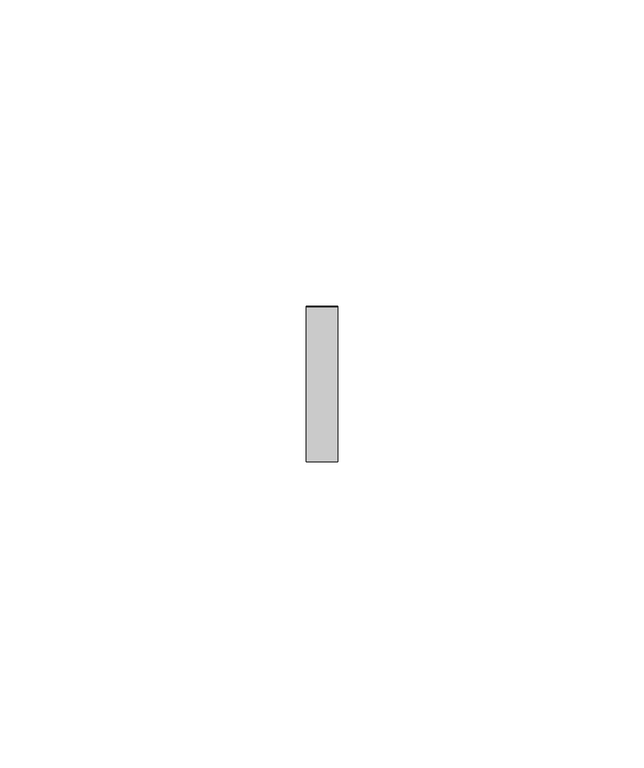
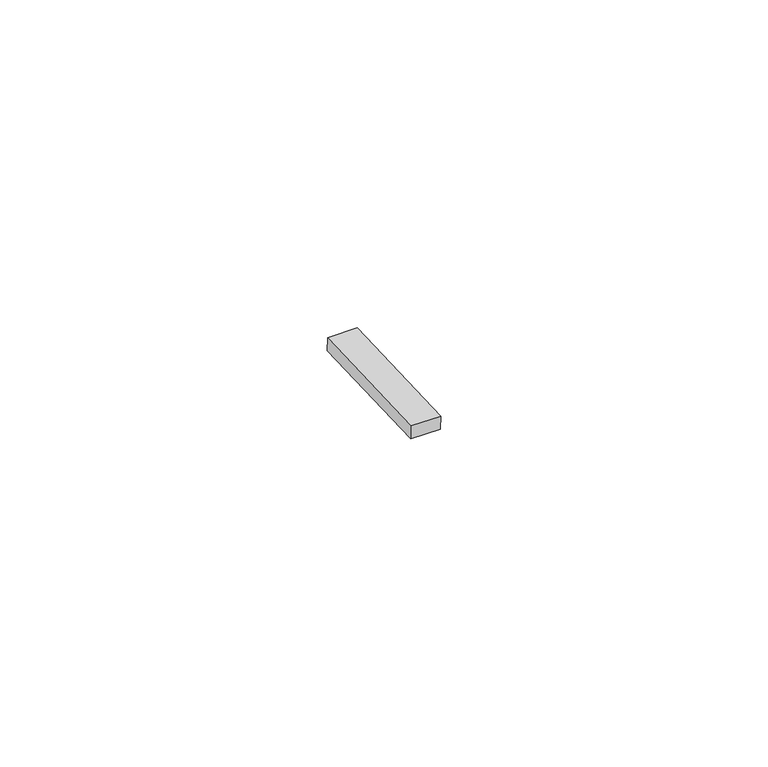
"""IFC4 building model written with IfcOpenShell, lengths in millimetres: proxy geometry, Inner panel:Inner panel:1:Inner panel:1 : Inner panel:Inner panel:300324:2:Inner panel:1:Inner panel:1 : Inner panel:Inner panel:300324:2 : Inner panel:Inner panel:1:Inner panel:1 : Inner panel:Inner panel:300324:300043:115 : Inner panel:Inner panel:1:Inner panel:1 : Inner panel:Inner panel:300324:2:Inner panel:1:Inner panel:1 : Inner panel:Inner panel:300324:2 : Inner panel:Inner panel:1:Inner panel:1 : Inner panel:Inner panel:300324:300043:308120."""

from ifc_helpers import new_model, si_unit, frame, origin, place, context, project, spatial, polyline, outline, extrude, source, transform, mapped, element, save


def generic_models_5e887ab9(model_context):
    return source(origin(), model_context, "Body", "SweptSolid", [
        extrude(outline(polyline([(0.0, -25.4), (0.0, 0.0), (5.2138089, 0.0), (5.2138089, -25.4), (0.0, -25.4)])), frame((593936.595117, -576574.3073926, 4050.9976844), z_axis=(0.0, -0.041630544712223896, 0.9991330730923502), x_axis=(-1.0, 0.0, 0.0)), (0.0, 0.0, 1.0), 2.4763745),
    ])


if __name__ == "__main__":
    model = new_model("IFC4")
    model_context = context("Model", 3, world=origin())
    ifc_project = project(units=[si_unit("LENGTHUNIT", "METRE", prefix="MILLI")], contexts=[model_context])
    site = spatial("IfcSite", under=ifc_project)
    building = spatial("IfcBuilding", under=site)
    placement = place(None, origin())
    generic_models_shape = generic_models_5e887ab9(model_context)
    element("IfcBuildingElementProxy", 1, Name="Inner panel:Inner panel:1:Inner panel:1 : Inner panel:Inner panel:300324:2:Inner panel:1:Inner panel:1 : Inner panel:Inner panel:300324:2 : Inner panel:Inner panel:1:Inner panel:1 : Inner panel:Inner panel:300324:300043:115 : Inner panel:Inner panel:1:Inner panel:1 : Inner panel:Inner panel:300324:2:Inner panel:1:Inner panel:1 : Inner panel:Inner panel:300324:2 : Inner panel:Inner panel:1:Inner panel:1 : Inner panel:Inner panel:300324:300043:308120", ObjectType="Inner panel:Inner panel:1:Inner panel:1 : Inner panel:Inner panel:300324:2:Inner panel:1:Inner panel:1 : Inner panel:Inner panel:300324:2 : Inner panel:Inner panel:1:Inner panel:1 : Inner panel:Inner panel:300324:300043:115 : Inner panel:Inner panel:1:Inner panel:1 : Inner panel:Inner panel:300324:2:Inner panel:1:Inner panel:1 : Inner panel:Inner panel:300324:2 : Inner panel:Inner panel:1:Inner panel:1 : Inner panel:Inner panel:300324:300043:308120", at=placement, inside=building, context=model_context, shape_type="MappedRepresentation", body=[
        mapped(generic_models_shape, transform((0.0, 0.0, 0.0), x_axis=(1.0, 0.0, 0.0), y_axis=(0.0, 1.0, 0.0), z_axis=(0.0, 0.0, 1.0))),
    ])
    save(model, "model.ifc")

# Revit data of these elements
# Type "Inner panel:Inner panel:1:Inner panel:1 : Inner panel:Inner panel:300324:2:Inner panel:1:Inner panel:1 : Inner panel:Inner panel:300324:2 : Inner panel:Inner panel:1:Inner panel:1 : Inner panel:Inner panel:300324:300043:115 : Inner panel:Inner panel:1:Inner panel:1 : Inner panel:Inner panel:300324:2:Inner panel:1:Inner panel:1 : Inner panel:Inner panel:300324:2 : Inner panel:Inner panel:1:Inner panel:1 : Inner panel:Inner panel:300324:300043:308120"
#   NameOverride = "Inner panel:Inner panel:1:Inner panel:1 : Inner panel:Inner panel:300324:2:Inner panel:1:Inner panel:1 : Inner panel:Inner panel:300324:2 : Inner panel:Inner panel:1:Inner panel:1 : Inner panel:Inner panel:300324:300043:308120"
#   ObjectTypeOverride = "Inner panel:1:Inner panel:1 : Inner panel:Inner panel:300324:2 : Inner panel:Inner panel:1:Inner panel:1 : Inner panel:Inner panel:300324:300043"
#   Reference = "Inner panel"
#   Tag = "308120"
# Element 1 (IfcBuildingElementProxy, "Inner panel:Inner panel:1:Inner panel:1 : Inner panel:Inner panel:300324:2:Inner panel:1:Inner panel:1 : Inner panel:Inner panel:300324:2 : Inner panel:Inner panel:1:Inner panel:1 : Inner panel:Inner panel:300324:300043:115 : Inner panel:Inner panel:1:Inner panel:1 : Inner panel:Inner panel:300324:2:Inner panel:1:Inner panel:1 : Inner panel:Inner panel:300324:2 : Inner panel:Inner panel:1:Inner panel:1 : Inner panel:Inner panel:300324:300043:308120")
#   Materials on its faces: "AT CLIP - 1\" WIDE NON ABSORBENT, WEATHER-RESISTANT NEOPRENE/EPDM/SBR FOAM"
# Materials
#   "AT CLIP - 1\" WIDE NON ABSORBENT, WEATHER-RESISTANT NEOPRENE/EPDM/SBR FOAM": class "Generic", colour RGB 85 85 85, transparency 0, Cost = 0
